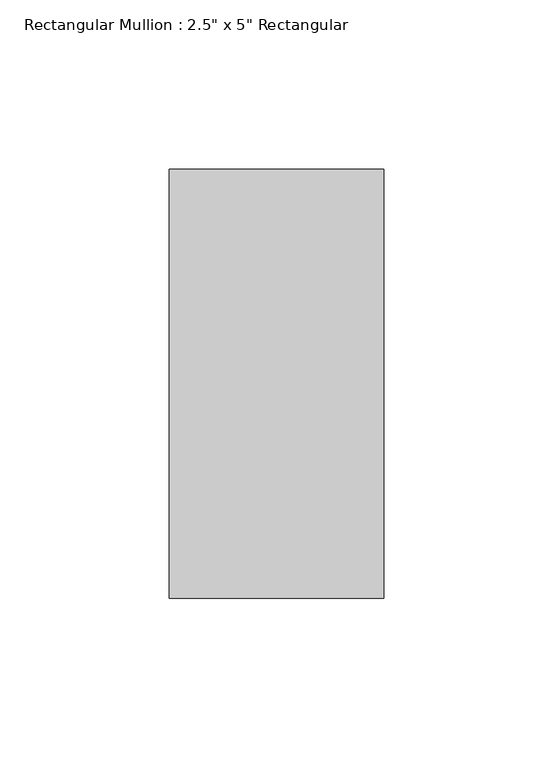
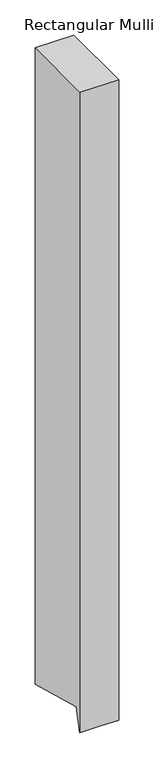
"""IFC4 building model written with IfcOpenShell, lengths in millimetres: member geometry."""

import ifcopenshell
import ifcopenshell.guid

model = None  # the IFC model being written
_history = None  # IfcOwnerHistory: only IFC2X3 demands one
_inside = {}  # id of a spatial element -> (the spatial element, [elements in it])
_under = {}  # id of a project, library or spatial element -> (it, [spatial elements below it])
_declared = {}  # id of a project -> (the project, [libraries it declares])
_typed = {}  # id of a type object -> (the type object, [elements of that type])
_made_of = {}  # id of a material, layer set ... -> (it, [elements and type objects made of it])


def new_model(schema):
    """Start an empty IFC model of exactly this schema.

    Asked for "IFC4X3", IfcOpenShell would pick the latest addendum, in which some entities
    have other attributes; the version numbers below select the first issue.
    IFC2X3 requires an IfcOwnerHistory on every rooted entity: one is made here for all.
    """
    global model, _history
    if schema == "IFC4X3":
        model = ifcopenshell.file(schema_version=(4, 3, 0, 0))
    else:
        model = ifcopenshell.file(schema=schema)
    _inside.clear()
    _under.clear()
    _declared.clear()
    _typed.clear()
    _made_of.clear()
    _history = None
    if model.schema == "IFC2X3":
        org = make("IfcOrganization", Name="unknown")
        user = make(
            "IfcPersonAndOrganization",
            ThePerson=make("IfcPerson", FamilyName="unknown"),
            TheOrganization=org,
        )
        app = make(
            "IfcApplication",
            ApplicationDeveloper=org,
            Version="unknown",
            ApplicationFullName="unknown",
            ApplicationIdentifier="unknown",
        )
        _history = make(
            "IfcOwnerHistory",
            OwningUser=user,
            OwningApplication=app,
            ChangeAction="ADDED",
            CreationDate=0,
        )
    return model


def make(cls, **values):
    """One entity of the class cls with the attributes given. An attribute that is None is left unset."""
    return model.create_entity(
        cls, **{name: value for name, value in values.items() if value is not None}
    )


def rooted(cls, **values):
    """An entity with a GlobalId (a new one), such as an element, a storey or a relation."""
    return make(cls, GlobalId=ifcopenshell.guid.new(), OwnerHistory=_history, **values)


def si_unit(unit_type, name, prefix=None):
    """IfcSIUnit, for example si_unit("LENGTHUNIT", "METRE", prefix="MILLI")."""
    return make("IfcSIUnit", UnitType=unit_type, Prefix=prefix, Name=name)


def assignment(units):
    """IfcUnitAssignment: the units of a project."""
    return None if units is None else make("IfcUnitAssignment", Units=units)


def point(xyz):
    """IfcCartesianPoint."""
    return None if xyz is None else make("IfcCartesianPoint", Coordinates=xyz)


def direction(xyz):
    """IfcDirection."""
    return None if xyz is None else make("IfcDirection", DirectionRatios=xyz)


def frame(location, z_axis=None, x_axis=None):
    """IfcAxis2Placement3D, a coordinate frame: its origin and axes. An axis left out is left unset."""
    return make(
        "IfcAxis2Placement3D",
        Location=point(location),
        Axis=direction(z_axis),
        RefDirection=direction(x_axis),
    )


def origin():
    """The frame at (0, 0, 0) with its axes left unset."""
    return frame((0.0, 0.0, 0.0))


def place(relative_to, where):
    """IfcLocalPlacement: puts the frame where relative to a parent placement (None: the world)."""
    return make(
        "IfcLocalPlacement", PlacementRelTo=relative_to, RelativePlacement=where
    )


def context(
    kind, dimensions, precision=None, world=None, true_north=None, identifier=None
):
    """IfcGeometricRepresentationContext, for example the 3D "Model" context."""
    return make(
        "IfcGeometricRepresentationContext",
        ContextIdentifier=identifier,
        ContextType=kind,
        CoordinateSpaceDimension=dimensions,
        Precision=precision,
        WorldCoordinateSystem=world,
        TrueNorth=true_north,
    )


def project(units=None, contexts=None):
    """IfcProject with its units and contexts."""
    return rooted(
        "IfcProject",
        Name="project",
        RepresentationContexts=contexts,
        UnitsInContext=assignment(units),
    )


def spatial(cls, under=None, at=None, **own):
    """A site, building, storey or space (cls), placed at a placement, below another one or the project."""
    s = rooted(cls, ObjectPlacement=at, **own)
    if under is not None:
        _under.setdefault(under.id(), (under, []))[1].append(s)
    return s


def faces_of(points, faces, orient=None, outer=None):
    """IfcFace entities. A face is a list of loops; a loop is a list of indices into points, from 0.

    orient and outer hold one flag for each loop. By default every Orientation is true, the
    first loop of a face is its IfcFaceOuterBound and the others are IfcFaceBound.
    """
    made = []
    for i, loops in enumerate(faces):
        bounds = []
        for j, loop in enumerate(loops):
            is_outer = j == 0 if outer is None else outer[i][j]
            bounds.append(
                make(
                    "IfcFaceOuterBound" if is_outer else "IfcFaceBound",
                    Bound=make("IfcPolyLoop", Polygon=[points[k] for k in loop]),
                    Orientation=True if orient is None else orient[i][j],
                )
            )
        made.append(make("IfcFace", Bounds=bounds))
    return made


def faceted_brep(points, faces, orient=None, outer=None, voids=None):
    """IfcFacetedBrep: a solid bounded by flat faces; with voids (closed shells), ...WithVoids."""
    shared = [point(p) for p in points]
    hull = make("IfcClosedShell", CfsFaces=faces_of(shared, faces, orient, outer))
    if voids is None:
        return make("IfcFacetedBrep", Outer=hull)
    return make(
        "IfcFacetedBrepWithVoids",
        Outer=hull,
        Voids=[
            make(cls, CfsFaces=faces_of(shared, fs, o, b)) for cls, fs, o, b in voids
        ],
    )


def shape(context_of_items, identifier, shape_type, items):
    """IfcShapeRepresentation: the items that make up one representation, for example the "Body"."""
    return make(
        "IfcShapeRepresentation",
        ContextOfItems=context_of_items,
        RepresentationIdentifier=identifier,
        RepresentationType=shape_type,
        Items=items,
    )


def source(mapping_origin, context_of_items, identifier, shape_type, items):
    """IfcRepresentationMap: a shape defined once, which mapped items show again and again."""
    return make(
        "IfcRepresentationMap",
        MappingOrigin=mapping_origin,
        MappedRepresentation=shape(context_of_items, identifier, shape_type, items),
    )


def transform(
    local_origin,
    x_axis=None,
    y_axis=None,
    z_axis=None,
    scale=None,
    scale2=None,
    scale3=None,
    uniform=True,
):
    """IfcCartesianTransformationOperator3D, or its non-uniform kind. x_axis, y_axis, z_axis: its Axis1, 2, 3."""
    if uniform:
        return make(
            "IfcCartesianTransformationOperator3D",
            Axis1=direction(x_axis),
            Axis2=direction(y_axis),
            LocalOrigin=point(local_origin),
            Scale=scale,
            Axis3=direction(z_axis),
        )
    return make(
        "IfcCartesianTransformationOperator3DnonUniform",
        Axis1=direction(x_axis),
        Axis2=direction(y_axis),
        LocalOrigin=point(local_origin),
        Scale=scale,
        Axis3=direction(z_axis),
        Scale2=scale2,
        Scale3=scale3,
    )


def mapped(mapping_source, mapping_target):
    """IfcMappedItem: shows the shape of a source again, moved by a transform."""
    return make(
        "IfcMappedItem", MappingSource=mapping_source, MappingTarget=mapping_target
    )


def made_of(thing, what):
    """Note that an element or type object is made of a material, layer set ...; save() writes the relation."""
    if what is not None:
        _made_of.setdefault(what.id(), (what, []))[1].append(thing)
    return thing


def element(
    cls,
    number,
    at=None,
    inside=None,
    cuts=None,
    type_object=None,
    material=None,
    context=None,
    identifier="Body",
    shape_type=None,
    held_by="IfcProductDefinitionShape",
    body=None,
    shapes=None,
    **own,
):
    """One element of the class cls, such as IfcWall. Its Tag is "e" and its number.

    at: its placement. inside: the storey or other place that contains it. cuts: it is an
    opening in that element (IfcRelVoidsElement). A single representation is given by context,
    identifier, shape_type and body (its items); several are given by shapes. held_by: the class
    of the entity that holds the representations. save() writes the other relations.
    """
    e = rooted(cls, Tag="e%d" % number, ObjectPlacement=at, **own)
    if body is not None:
        shapes = [shape(context, identifier, shape_type, body)]
    if shapes is not None:
        e.Representation = make(held_by, Representations=shapes)
    if inside is not None:
        _inside.setdefault(inside.id(), (inside, []))[1].append(e)
    if cuts is not None:
        rooted(
            "IfcRelVoidsElement", RelatingBuildingElement=cuts, RelatedOpeningElement=e
        )
    if type_object is not None:
        _typed.setdefault(type_object.id(), (type_object, []))[1].append(e)
    return made_of(e, material)


def aggregate(whole, parts):
    """IfcRelAggregates: a whole, such as a stair, and the parts it consists of."""
    return rooted("IfcRelAggregates", RelatingObject=whole, RelatedObjects=parts)


def save(model, path):
    """Write the relations noted so far, then the file.

    IfcRelAggregates (storeys below a building ...), IfcRelContainedInSpatialStructure (elements
    in a storey), IfcRelDefinesByType, IfcRelAssociatesMaterial and IfcRelDeclares: one each for
    every whole, place, type object, material and project.
    """
    for whole, parts in _under.values():
        aggregate(whole, parts)
    for where, things in _inside.values():
        rooted(
            "IfcRelContainedInSpatialStructure",
            RelatedElements=things,
            RelatingStructure=where,
        )
    for kind, things in _typed.values():
        rooted("IfcRelDefinesByType", RelatedObjects=things, RelatingType=kind)
    for what, things in _made_of.values():
        rooted("IfcRelAssociatesMaterial", RelatedObjects=things, RelatingMaterial=what)
    for by, libraries in _declared.values():
        rooted("IfcRelDeclares", RelatingContext=by, RelatedDefinitions=libraries)
    model.write(path)


def member_00117584(model_context):
    return source(origin(), model_context, "Body", "Brep", [
        faceted_brep([(31.75, 63.5, 0.0), (-31.75, 63.5, 0.0), (-31.75, -63.5, 0.0), (31.75, -63.5, 0.0), (31.75, 63.5, -1103.9654292), (0.0, 63.5, -1103.9654292), (-31.75, 63.5, -1103.9654292), (-31.75, -53.1187853, -1072.7175199), (-31.75, -63.5, -1111.4607406), (0.0, -63.5, -1111.4607406), (31.75, -63.5, -1111.4607406), (31.75, -53.1187853, -1072.7175199), (0.0, -53.1187853, -1072.7175199)], [[[0, 1, 2, 3]], [[1, 0, 4, 5, 6]], [[2, 1, 6, 7, 8]], [[3, 2, 8, 9, 10]], [[0, 3, 10, 11, 4]], [[4, 11, 12, 5]], [[11, 10, 9, 12]], [[9, 8, 7, 12]], [[7, 6, 5, 12]]]),
    ])


if __name__ == "__main__":
    model = new_model("IFC4")
    model_context = context("Model", 3, world=origin())
    ifc_project = project(units=[si_unit("LENGTHUNIT", "METRE", prefix="MILLI")], contexts=[model_context])
    site = spatial("IfcSite", under=ifc_project)
    building = spatial("IfcBuilding", under=site)
    placement = place(None, origin())
    member_shape = member_00117584(model_context)
    element("IfcMember", 1, ObjectType="Rectangular Mullion : 2.5\" x 5\" Rectangular", at=placement, inside=building, context=model_context, shape_type="MappedRepresentation", body=[
        mapped(member_shape, transform((0.0, 0.0, 0.0), x_axis=(1.0, 0.0, 0.0), y_axis=(0.0, 1.0, 0.0), z_axis=(0.0, 0.0, 1.0))),
    ])
    save(model, "model.ifc")

# Revit data of these elements
# Project information
#   Project Issue Date = "Issue Date"
#   Project Status = "Project Status"
#   Client Name = "Owner"
#   Project Address = "Enter address here"
#   Project Name = "Project Name"
#   Project Number = "Project Number"
# Type "Rectangular Mullion : 2.5\" x 5\" Rectangular"
#   built-in parameter 1007304 = 0.416667 (stored number, unit not read)
#   built-in parameter 1007301 = 0.104167 (stored number, unit not read)
#   built-in parameter 1007300 = 0.104167 (stored number, unit not read)
# Element 1 (IfcMember, "Rectangular Mullion : 2.5\" x 5\" Rectangular")
#   Materials on its faces: "Aluminum"
# Materials
#   "Aluminum": class "Metal", colour RGB 247 247 247, transparency 0, Description = "Aluminum 6061", Cost = 0
